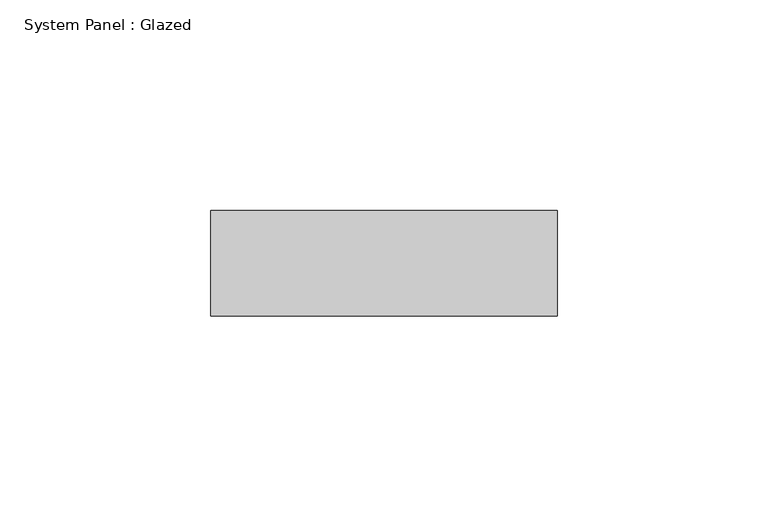
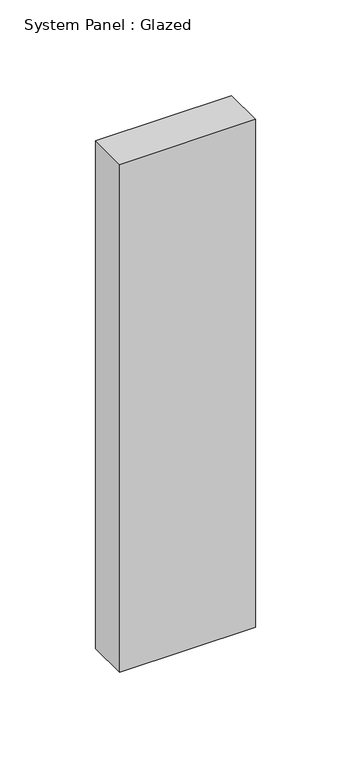
"""IFC4 building model written with IfcOpenShell, lengths in millimetres: plate geometry, System Panel : Glazed."""

from ifc_helpers import new_model, si_unit, origin, origin_with_axes, place, context, project, spatial, polyline, outline, extrude, source, transform, mapped, element, save


def system_panel_glazed_3cd50573(model_context):
    return source(origin(), model_context, "Body", "SweptSolid", [
        extrude(outline(polyline([(41.0454544, 24.5), (-41.0454544, 24.5), (-41.0454544, 49.5), (41.0454544, 49.5), (41.0454544, 24.5)])), origin_with_axes(), (0.0, 0.0, 1.0), 323.8777657),
    ])


if __name__ == "__main__":
    model = new_model("IFC4")
    model_context = context("Model", 3, world=origin())
    ifc_project = project(units=[si_unit("LENGTHUNIT", "METRE", prefix="MILLI")], contexts=[model_context])
    site = spatial("IfcSite", under=ifc_project)
    building = spatial("IfcBuilding", under=site)
    placement = place(None, origin())
    system_panel_glazed_shape = system_panel_glazed_3cd50573(model_context)
    element("IfcPlate", 1, ObjectType="System Panel : Glazed", at=placement, inside=building, context=model_context, shape_type="MappedRepresentation", body=[
        mapped(system_panel_glazed_shape, transform((0.0, 0.0, 0.0), x_axis=(1.0, 0.0, 0.0), y_axis=(0.0, 1.0, 0.0), z_axis=(0.0, 0.0, 1.0))),
    ])
    save(model, "model.ifc")

# Revit data of these elements
# Element 1 (IfcPlate, "System Panel : Glazed")
#   Materials on its faces: "Glass"
# Materials
#   "Glass": class "Glass", colour RGB 218 227 224, transparency 0.85, Description = "Soda Lime Glass", Cost = 0
